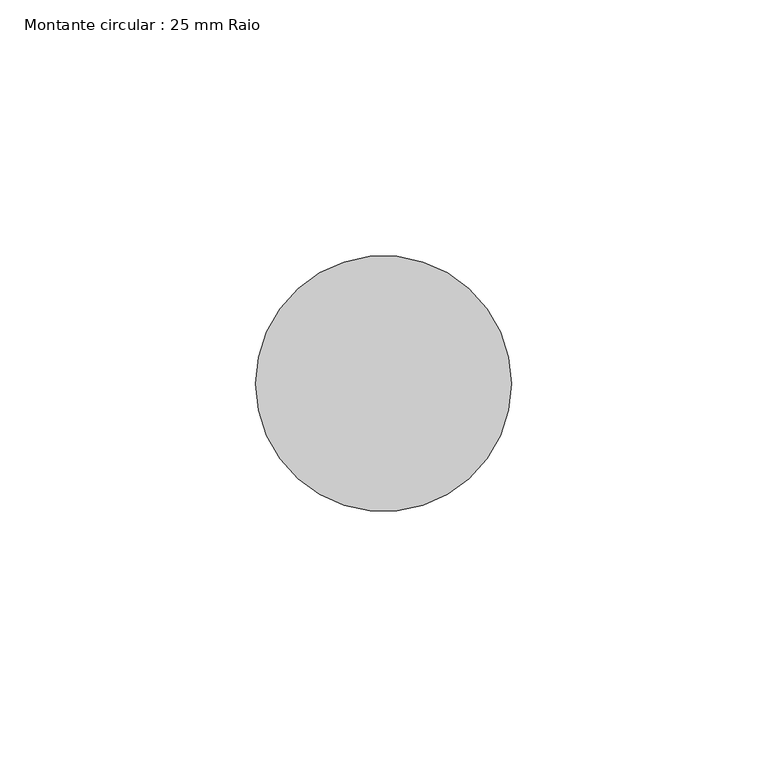
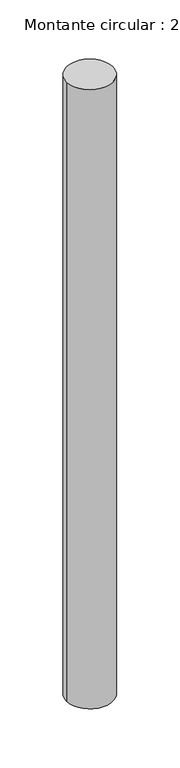
"""IFC4 building model written with IfcOpenShell, lengths in millimetres: member geometry, Montante circular : 25 mm Raio."""

from ifc_helpers import new_model, si_unit, point, frame, origin, origin_2d, place, context, project, spatial, circle_curve, trimmed, segment, composite_curve, outline, extrude, source, transform, mapped, element, save


def montante_circular_25_mm_raio_1abe9a59(model_context):
    return source(origin(), model_context, "Body", "SweptSolid", [
        extrude(outline(composite_curve([segment(trimmed(circle_curve(origin_2d(), 25.0), [point((25.0, 0.0))], [point((-25.0, 0.0))], False, "CARTESIAN"), True, "CONTINUOUS"), segment(trimmed(circle_curve(origin_2d(), 25.0), [point((-25.0, 0.0))], [point((25.0, 0.0))], False, "CARTESIAN"), True, "CONTINUOUS")], self_intersect=False)), frame((0.0, 0.0, -706.665615), z_axis=(0.0, 0.0, 1.0), x_axis=(1.0, 0.0, 0.0)), (0.0, 0.0, 1.0), 706.665615),
    ])


if __name__ == "__main__":
    model = new_model("IFC4")
    model_context = context("Model", 3, world=origin())
    ifc_project = project(units=[si_unit("LENGTHUNIT", "METRE", prefix="MILLI")], contexts=[model_context])
    site = spatial("IfcSite", under=ifc_project)
    building = spatial("IfcBuilding", under=site)
    placement = place(None, origin())
    montante_circular_25_mm_raio_shape = montante_circular_25_mm_raio_1abe9a59(model_context)
    element("IfcMember", 1, ObjectType="Montante circular : 25 mm Raio", at=placement, inside=building, context=model_context, shape_type="MappedRepresentation", body=[
        mapped(montante_circular_25_mm_raio_shape, transform((0.0, 0.0, 0.0), x_axis=(1.0, 0.0, 0.0), y_axis=(0.0, 1.0, 0.0), z_axis=(0.0, 0.0, 1.0))),
    ])
    save(model, "model.ifc")

# Revit data of these elements
# Type "Montante circular : 25 mm Raio"
#   built-in parameter 1007350 = 0.082021 (stored number, unit not read)
# Element 1 (IfcMember, "Montante circular : 25 mm Raio")
#   Materials on its faces: "Alumín."
# Materials
#   "Alumín.": class "Metal", colour RGB 247 247 247, transparency 0, Description = "Alumín. 6061", Cost = 0
